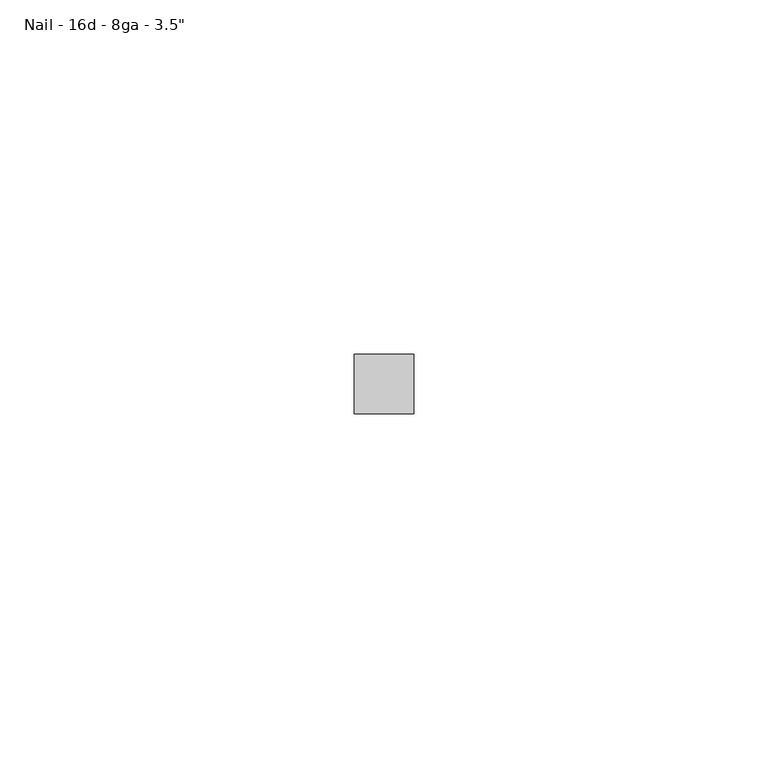
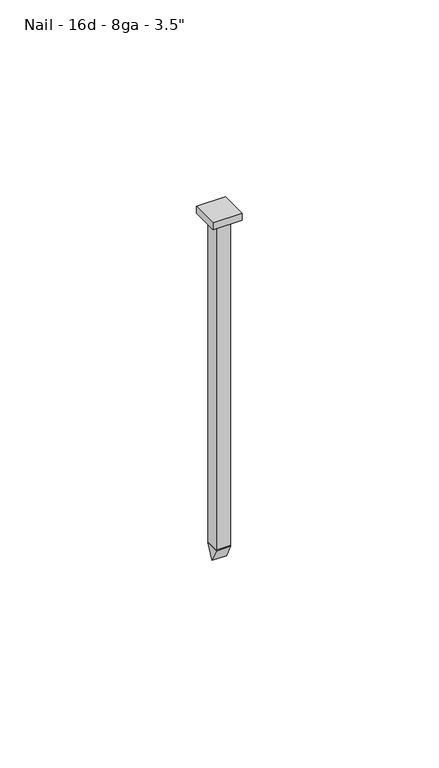
"""IFC4 building model written with IfcOpenShell, lengths in millimetres: fastener geometry."""

import ifcopenshell
import ifcopenshell.guid

model = None  # the IFC model being written
_history = None  # IfcOwnerHistory: only IFC2X3 demands one
_inside = {}  # id of a spatial element -> (the spatial element, [elements in it])
_under = {}  # id of a project, library or spatial element -> (it, [spatial elements below it])
_declared = {}  # id of a project -> (the project, [libraries it declares])
_typed = {}  # id of a type object -> (the type object, [elements of that type])
_made_of = {}  # id of a material, layer set ... -> (it, [elements and type objects made of it])


def new_model(schema):
    """Start an empty IFC model of exactly this schema.

    Asked for "IFC4X3", IfcOpenShell would pick the latest addendum, in which some entities
    have other attributes; the version numbers below select the first issue.
    IFC2X3 requires an IfcOwnerHistory on every rooted entity: one is made here for all.
    """
    global model, _history
    if schema == "IFC4X3":
        model = ifcopenshell.file(schema_version=(4, 3, 0, 0))
    else:
        model = ifcopenshell.file(schema=schema)
    _inside.clear()
    _under.clear()
    _declared.clear()
    _typed.clear()
    _made_of.clear()
    _history = None
    if model.schema == "IFC2X3":
        org = make("IfcOrganization", Name="unknown")
        user = make(
            "IfcPersonAndOrganization",
            ThePerson=make("IfcPerson", FamilyName="unknown"),
            TheOrganization=org,
        )
        app = make(
            "IfcApplication",
            ApplicationDeveloper=org,
            Version="unknown",
            ApplicationFullName="unknown",
            ApplicationIdentifier="unknown",
        )
        _history = make(
            "IfcOwnerHistory",
            OwningUser=user,
            OwningApplication=app,
            ChangeAction="ADDED",
            CreationDate=0,
        )
    return model


def make(cls, **values):
    """One entity of the class cls with the attributes given. An attribute that is None is left unset."""
    return model.create_entity(
        cls, **{name: value for name, value in values.items() if value is not None}
    )


def rooted(cls, **values):
    """An entity with a GlobalId (a new one), such as an element, a storey or a relation."""
    return make(cls, GlobalId=ifcopenshell.guid.new(), OwnerHistory=_history, **values)


def si_unit(unit_type, name, prefix=None):
    """IfcSIUnit, for example si_unit("LENGTHUNIT", "METRE", prefix="MILLI")."""
    return make("IfcSIUnit", UnitType=unit_type, Prefix=prefix, Name=name)


def assignment(units):
    """IfcUnitAssignment: the units of a project."""
    return None if units is None else make("IfcUnitAssignment", Units=units)


def point(xyz):
    """IfcCartesianPoint."""
    return None if xyz is None else make("IfcCartesianPoint", Coordinates=xyz)


def direction(xyz):
    """IfcDirection."""
    return None if xyz is None else make("IfcDirection", DirectionRatios=xyz)


def frame(location, z_axis=None, x_axis=None):
    """IfcAxis2Placement3D, a coordinate frame: its origin and axes. An axis left out is left unset."""
    return make(
        "IfcAxis2Placement3D",
        Location=point(location),
        Axis=direction(z_axis),
        RefDirection=direction(x_axis),
    )


def origin():
    """The frame at (0, 0, 0) with its axes left unset."""
    return frame((0.0, 0.0, 0.0))


def origin_with_axes():
    """The frame at (0, 0, 0) with the z axis (0, 0, 1) and the x axis (1, 0, 0) written out."""
    return frame((0.0, 0.0, 0.0), z_axis=(0.0, 0.0, 1.0), x_axis=(1.0, 0.0, 0.0))


def place(relative_to, where):
    """IfcLocalPlacement: puts the frame where relative to a parent placement (None: the world)."""
    return make(
        "IfcLocalPlacement", PlacementRelTo=relative_to, RelativePlacement=where
    )


def context(
    kind, dimensions, precision=None, world=None, true_north=None, identifier=None
):
    """IfcGeometricRepresentationContext, for example the 3D "Model" context."""
    return make(
        "IfcGeometricRepresentationContext",
        ContextIdentifier=identifier,
        ContextType=kind,
        CoordinateSpaceDimension=dimensions,
        Precision=precision,
        WorldCoordinateSystem=world,
        TrueNorth=true_north,
    )


def project(units=None, contexts=None):
    """IfcProject with its units and contexts."""
    return rooted(
        "IfcProject",
        Name="project",
        RepresentationContexts=contexts,
        UnitsInContext=assignment(units),
    )


def spatial(cls, under=None, at=None, **own):
    """A site, building, storey or space (cls), placed at a placement, below another one or the project."""
    s = rooted(cls, ObjectPlacement=at, **own)
    if under is not None:
        _under.setdefault(under.id(), (under, []))[1].append(s)
    return s


def polyline(points):
    """IfcPolyline through the points."""
    return make("IfcPolyline", Points=[point(p) for p in points])


def outline(outer, holes=None, kind="AREA"):
    """IfcArbitraryClosedProfileDef: a profile drawn as a closed curve; with holes, ...WithVoids."""
    if holes is None:
        return make("IfcArbitraryClosedProfileDef", ProfileType=kind, OuterCurve=outer)
    return make(
        "IfcArbitraryProfileDefWithVoids",
        ProfileType=kind,
        OuterCurve=outer,
        InnerCurves=holes,
    )


def extrude(swept, where, along, depth):
    """IfcExtrudedAreaSolid: the profile swept, set in the frame where, extruded along a direction by depth."""
    return make(
        "IfcExtrudedAreaSolid",
        SweptArea=swept,
        Position=where,
        ExtrudedDirection=direction(along),
        Depth=depth,
    )


def shape(context_of_items, identifier, shape_type, items):
    """IfcShapeRepresentation: the items that make up one representation, for example the "Body"."""
    return make(
        "IfcShapeRepresentation",
        ContextOfItems=context_of_items,
        RepresentationIdentifier=identifier,
        RepresentationType=shape_type,
        Items=items,
    )


def source(mapping_origin, context_of_items, identifier, shape_type, items):
    """IfcRepresentationMap: a shape defined once, which mapped items show again and again."""
    return make(
        "IfcRepresentationMap",
        MappingOrigin=mapping_origin,
        MappedRepresentation=shape(context_of_items, identifier, shape_type, items),
    )


def transform(
    local_origin,
    x_axis=None,
    y_axis=None,
    z_axis=None,
    scale=None,
    scale2=None,
    scale3=None,
    uniform=True,
):
    """IfcCartesianTransformationOperator3D, or its non-uniform kind. x_axis, y_axis, z_axis: its Axis1, 2, 3."""
    if uniform:
        return make(
            "IfcCartesianTransformationOperator3D",
            Axis1=direction(x_axis),
            Axis2=direction(y_axis),
            LocalOrigin=point(local_origin),
            Scale=scale,
            Axis3=direction(z_axis),
        )
    return make(
        "IfcCartesianTransformationOperator3DnonUniform",
        Axis1=direction(x_axis),
        Axis2=direction(y_axis),
        LocalOrigin=point(local_origin),
        Scale=scale,
        Axis3=direction(z_axis),
        Scale2=scale2,
        Scale3=scale3,
    )


def mapped(mapping_source, mapping_target):
    """IfcMappedItem: shows the shape of a source again, moved by a transform."""
    return make(
        "IfcMappedItem", MappingSource=mapping_source, MappingTarget=mapping_target
    )


def made_of(thing, what):
    """Note that an element or type object is made of a material, layer set ...; save() writes the relation."""
    if what is not None:
        _made_of.setdefault(what.id(), (what, []))[1].append(thing)
    return thing


def element(
    cls,
    number,
    at=None,
    inside=None,
    cuts=None,
    type_object=None,
    material=None,
    context=None,
    identifier="Body",
    shape_type=None,
    held_by="IfcProductDefinitionShape",
    body=None,
    shapes=None,
    **own,
):
    """One element of the class cls, such as IfcWall. Its Tag is "e" and its number.

    at: its placement. inside: the storey or other place that contains it. cuts: it is an
    opening in that element (IfcRelVoidsElement). A single representation is given by context,
    identifier, shape_type and body (its items); several are given by shapes. held_by: the class
    of the entity that holds the representations. save() writes the other relations.
    """
    e = rooted(cls, Tag="e%d" % number, ObjectPlacement=at, **own)
    if body is not None:
        shapes = [shape(context, identifier, shape_type, body)]
    if shapes is not None:
        e.Representation = make(held_by, Representations=shapes)
    if inside is not None:
        _inside.setdefault(inside.id(), (inside, []))[1].append(e)
    if cuts is not None:
        rooted(
            "IfcRelVoidsElement", RelatingBuildingElement=cuts, RelatedOpeningElement=e
        )
    if type_object is not None:
        _typed.setdefault(type_object.id(), (type_object, []))[1].append(e)
    return made_of(e, material)


def aggregate(whole, parts):
    """IfcRelAggregates: a whole, such as a stair, and the parts it consists of."""
    return rooted("IfcRelAggregates", RelatingObject=whole, RelatedObjects=parts)


def save(model, path):
    """Write the relations noted so far, then the file.

    IfcRelAggregates (storeys below a building ...), IfcRelContainedInSpatialStructure (elements
    in a storey), IfcRelDefinesByType, IfcRelAssociatesMaterial and IfcRelDeclares: one each for
    every whole, place, type object, material and project.
    """
    for whole, parts in _under.values():
        aggregate(whole, parts)
    for where, things in _inside.values():
        rooted(
            "IfcRelContainedInSpatialStructure",
            RelatedElements=things,
            RelatingStructure=where,
        )
    for kind, things in _typed.values():
        rooted("IfcRelDefinesByType", RelatedObjects=things, RelatingType=kind)
    for what, things in _made_of.values():
        rooted("IfcRelAssociatesMaterial", RelatedObjects=things, RelatingMaterial=what)
    for by, libraries in _declared.values():
        rooted("IfcRelDeclares", RelatingContext=by, RelatedDefinitions=libraries)
    model.write(path)


def fastener_034bf7df(model_context):
    return source(origin(), model_context, "Body", "SweptSolid", [
        extrude(outline(polyline([(0.0, -105.791), (-2.0955, -101.6), (2.0955, -101.6), (0.0, -105.791)])), frame((-2.0955, 0.0, 0.0), z_axis=(1.0, 0.0, 0.0), x_axis=(0.0, 1.0, 0.0)), (0.0, 0.0, 1.0), 4.191),
        extrude(outline(polyline([(-4.191, -4.191), (-4.191, 4.191), (4.191, 4.191), (4.191, -4.191), (-4.191, -4.191)])), origin_with_axes(), (0.0, 0.0, 1.0), 2.0955),
        extrude(outline(polyline([(-2.0955, 2.0955), (2.0955, 2.0955), (2.0955, -2.0955), (-2.0955, -2.0955), (-2.0955, 2.0955)])), frame((0.0, 0.0, -101.6), z_axis=(0.0, 0.0, 1.0), x_axis=(1.0, 0.0, 0.0)), (0.0, 0.0, 1.0), 101.6),
    ])


if __name__ == "__main__":
    model = new_model("IFC4")
    model_context = context("Model", 3, world=origin())
    ifc_project = project(units=[si_unit("LENGTHUNIT", "METRE", prefix="MILLI")], contexts=[model_context])
    site = spatial("IfcSite", under=ifc_project)
    building = spatial("IfcBuilding", under=site)
    placement = place(None, origin())
    fastener_shape = fastener_034bf7df(model_context)
    element("IfcFastener", 1, ObjectType="060523 - W_P_C - Fastenings - Generic - SQUARE : Nail - 16d - 8ga - 3.5\"", at=placement, inside=building, context=model_context, shape_type="MappedRepresentation", body=[
        mapped(fastener_shape, transform((0.0, 0.0, 0.0), x_axis=(1.0, 0.0, 0.0), y_axis=(0.0, 1.0, 0.0), z_axis=(0.0, 0.0, 1.0))),
    ])
    save(model, "model.ifc")

# Revit data of these elements
# Type "060523 - W_P_C - Fastenings - Generic - SQUARE : Nail - 16d - 8ga - 3.5\""
#   Washer_Thickness = 0' - 0.00333"
#   Washer Radius = 0' - 0.0925"
#   Washer Offset - Head = 0' - 0"
#   Washer Offset = 0' - 0"
#   Thickness_of_Substrate [instance default] = 0' - 1"
#   Side = 0' - 0 37/64"
#   Radius = 0' - 0.0825"
#   Length [instance default] = 0' - 3 1/2"
#   Head Size = 0' - 1"
#   Head Radius = 0' - 0 1/2"
#   Head Height = 0' - 0.01"
#   Double Diameter = 0' - 0.33"
#   Diameter = 0' - 0.165"
#   Default Elevation = 4' - 0"
#   Washer_Nut_Visibility = no
#   Washer_Head_Visibility = no
#   Round_Head_Visibility = yes
#   Point Visibility = yes
#   Nut_Visibility = no
#   Hex_Head_Visiblilty = no
#   Washer Material = none
#   Bolt Material (Size) = AT SILL - FASTENER AT 24" O.C.
# Element 1 (IfcFastener, "060523 - W_P_C - Fastenings - Generic - SQUARE : Nail - 16d - 8ga - 3.5\"")
#   Length = 0' - 4"
# Materials
#   "AT SILL - FASTENER AT 24\" O.C.": class "Generic", colour RGB 120 120 120, transparency 0, Cost = 0
